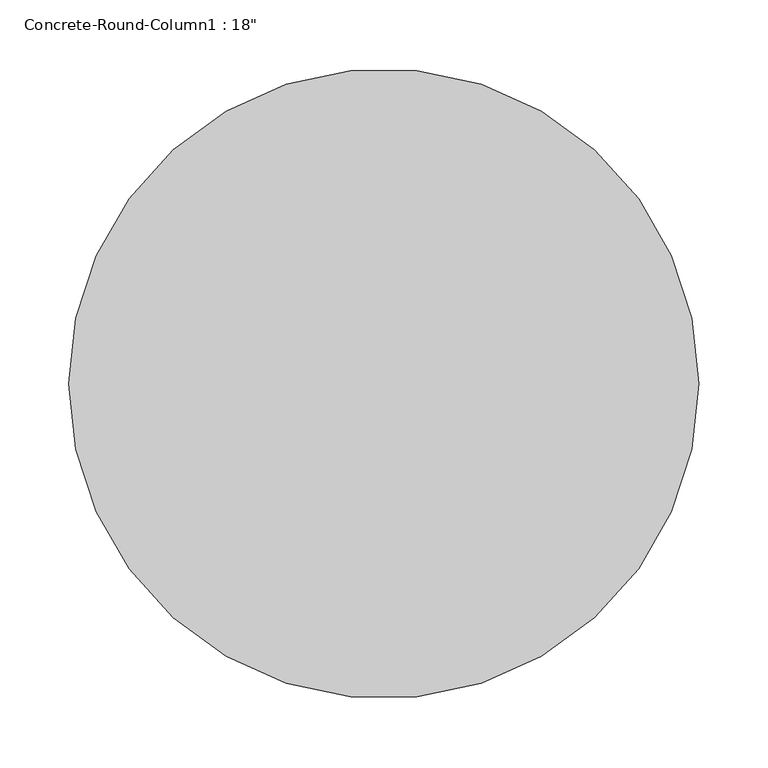
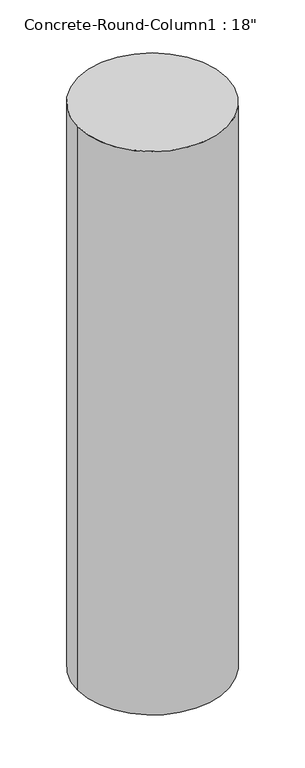
"""IFC4 building model written with IfcOpenShell, lengths in millimetres: column geometry."""

from ifc_helpers import new_model, si_unit, point, frame, origin, origin_2d, place, context, project, spatial, circle_curve, trimmed, segment, composite_curve, outline, extrude, source, transform, mapped, element, save


def column_5a4f3ead(model_context):
    return source(origin(), model_context, "Body", "SweptSolid", [
        extrude(outline(composite_curve([segment(trimmed(circle_curve(origin_2d(), 228.6), [point((-228.6, 0.0))], [point((228.6, 0.0))], False, "CARTESIAN"), True, "CONTINUOUS"), segment(trimmed(circle_curve(origin_2d(), 228.6), [point((228.6, 0.0))], [point((-228.6, 0.0))], False, "CARTESIAN"), True, "CONTINUOUS")], self_intersect=False)), frame((0.0, 0.0, -1219.2), z_axis=(0.0, 0.0, 1.0), x_axis=(1.0, 0.0, 0.0)), (0.0, 0.0, 1.0), 1828.8),
    ])


if __name__ == "__main__":
    model = new_model("IFC4")
    model_context = context("Model", 3, world=origin())
    ifc_project = project(units=[si_unit("LENGTHUNIT", "METRE", prefix="MILLI")], contexts=[model_context])
    site = spatial("IfcSite", under=ifc_project)
    building = spatial("IfcBuilding", under=site)
    placement = place(None, origin())
    column_shape = column_5a4f3ead(model_context)
    element("IfcColumn", 1, ObjectType="Concrete-Round-Column1 : 18\"", at=placement, inside=building, context=model_context, shape_type="MappedRepresentation", body=[
        mapped(column_shape, transform((0.0, 0.0, 0.0), x_axis=(1.0, 0.0, 0.0), y_axis=(0.0, 1.0, 0.0), z_axis=(0.0, 0.0, 1.0))),
    ])
    save(model, "model.ifc")

# Revit data of these elements
# Type "Concrete-Round-Column1 : 18\""
#   Assembly Code = "B10"
#   b = 1' - 6"
#   Column Material [instance default] = Concrete - Cast-in-Place Concrete
# Element 1 (IfcColumn, "Concrete-Round-Column1 : 18\"")
#   Materials on its faces: "Concrete - Cast-in-Place Concrete"
# Materials
#   "Concrete - Cast-in-Place Concrete": class "Concrete", colour RGB 192 192 192, transparency 0
